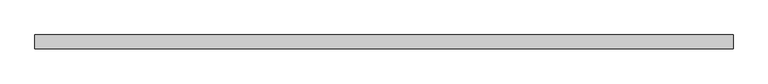
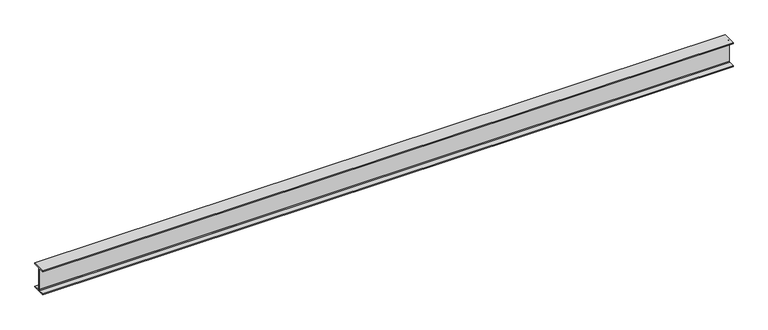
"""IFC4 building model written with IfcOpenShell, lengths in millimetres: beam geometry, Old_Steel Beam_H-KSD3502 : H_SB_ASB_H-340×250x9x14."""

from ifc_helpers import new_model, si_unit, point, frame, frame_2d, origin, place, context, project, spatial, polyline, circle_curve, trimmed, segment, composite_curve, outline, extrude, source, transform, mapped, element, save


def beam_27ecb92b(model_context):
    return source(origin(), model_context, "Body", "SweptSolid", [
        extrude(outline(composite_curve([segment(polyline([(82.5, -141.5), (82.5, -151.7), (-82.5, -151.7), (-82.5, -141.5), (-11.9, -141.5)]), True, "CONTINUOUS"), segment(trimmed(circle_curve(frame_2d((-11.9, -132.6)), 8.9), [point((-11.9, -141.5))], [point((-3.0, -132.6))], True, "CARTESIAN"), True, "CONTINUOUS"), segment(polyline([(-3.0, -132.6), (-3.0, 132.6)]), True, "CONTINUOUS"), segment(trimmed(circle_curve(frame_2d((-11.9, 132.6)), 8.9), [point((-3.0, 132.6))], [point((-11.9, 141.5))], True, "CARTESIAN"), True, "CONTINUOUS"), segment(polyline([(-11.9, 141.5), (-82.5, 141.5), (-82.5, 151.7), (82.5, 151.7), (82.5, 141.5), (11.9, 141.5)]), True, "CONTINUOUS"), segment(trimmed(circle_curve(frame_2d((11.9, 132.6)), 8.9), [point((11.9, 141.5))], [point((3.0, 132.6))], True, "CARTESIAN"), True, "CONTINUOUS"), segment(polyline([(3.0, 132.6), (3.0, -132.6)]), True, "CONTINUOUS"), segment(trimmed(circle_curve(frame_2d((11.9, -132.6)), 8.9), [point((3.0, -132.6))], [point((11.9, -141.5))], True, "CARTESIAN"), True, "CONTINUOUS"), segment(polyline([(11.9, -141.5), (82.5, -141.5)]), True, "CONTINUOUS")], self_intersect=False)), frame((-4154.8, 0.0, 0.0), z_axis=(1.0, 0.0, 0.0), x_axis=(0.0, 1.0, 0.0)), (0.0, 0.0, 1.0), 8309.6),
    ])


if __name__ == "__main__":
    model = new_model("IFC4")
    model_context = context("Model", 3, world=origin())
    ifc_project = project(units=[si_unit("LENGTHUNIT", "METRE", prefix="MILLI")], contexts=[model_context])
    site = spatial("IfcSite", under=ifc_project)
    building = spatial("IfcBuilding", under=site)
    placement = place(None, origin())
    beam_shape = beam_27ecb92b(model_context)
    element("IfcBeam", 1, ObjectType="Old_Steel Beam_H-KSD3502 : H_SB_ASB_H-340×250x9x14", at=placement, inside=building, context=model_context, shape_type="MappedRepresentation", body=[
        mapped(beam_shape, transform((0.0, 0.0, 0.0), x_axis=(1.0, 0.0, 0.0), y_axis=(0.0, 1.0, 0.0), z_axis=(0.0, 0.0, 1.0))),
    ])
    save(model, "model.ifc")

# Revit data of these elements
# Type "Old_Steel Beam_H-KSD3502 : H_SB_ASB_H-340×250x9x14"
#   Width = 25.0 cm
#   Web Thickness = 0.9 cm
#   Web Fillet = 2.0 cm
#   Warping Constant = 968661.0 cm⁶
#   Torsional Moment of Inertia = 53.6551 cm⁴
#   Torsional Modulus = 1.0 cm³
#   Section Area = 101.5 cm²
#   Plastic Modulus weak axis = 447.0 cm³
#   Plastic Modulus strong axis = 1410.0 cm³
#   Perimeter = 1.63 m²/m
#   Nominal Weight = 79.70 kgf/m
#   Moment of Inertia weak axis = 3650.00 cm⁴
#   Moment of Inertia strong axis = 21700.00 cm⁴
#   Height = 34.0 cm
#   Flange Thickness = 1.4 cm
#   Elastic Modulus weak axis = 292.0 cm³
#   Elastic Modulus strong axis = 1280.0 cm³
#   Centroid Vertical = 17.0 cm
#   Centroid Horizontal = 12.5 cm
#   Length [instance default] = 1.5240 m
#   Structural Material [instance default] = Steel, 45-345
#   Assembly Code = ""
# Element 1 (IfcBeam, "Old_Steel Beam_H-KSD3502 : H_SB_ASB_H-340×250x9x14")
#   Structural Material = none
# Materials
#   "Steel, 45-345": class "Metal", colour RGB 189 187 185, transparency 0, Description = "Steel 345 MPa", Cost = 0
